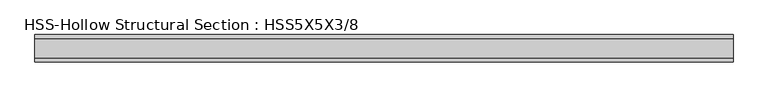
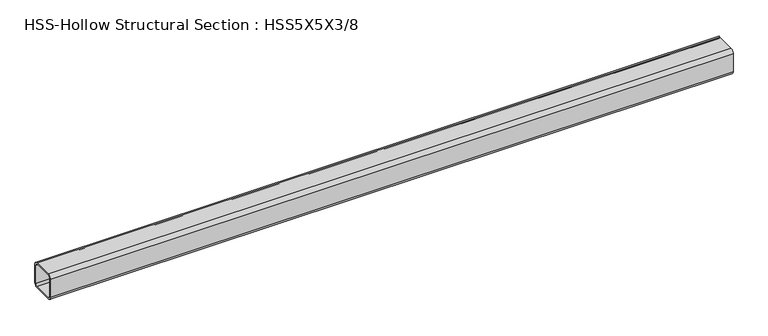
"""IFC4 building model written with IfcOpenShell, lengths in millimetres: member geometry, HSS-Hollow Structural Section : HSS5X5X3/8."""

from ifc_helpers import new_model, si_unit, point, frame, frame_2d, origin, place, context, project, spatial, polyline, circle_curve, trimmed, segment, composite_curve, outline, extrude, source, transform, mapped, element, save


def hss_hollow_structural_section_hss5x5x3_8_3ac4091e(model_context):
    return source(origin(), model_context, "Body", "SweptSolid", [
        extrude(outline(composite_curve([segment(polyline([(63.5, 45.7708), (63.5, -45.7708)]), True, "CONTINUOUS"), segment(trimmed(circle_curve(frame_2d((45.7708, -45.7708)), 17.7292), [point((63.5, -45.7708))], [point((45.7708, -63.5))], False, "CARTESIAN"), True, "CONTINUOUS"), segment(polyline([(45.7708, -63.5), (-45.7708, -63.5)]), True, "CONTINUOUS"), segment(trimmed(circle_curve(frame_2d((-45.7708, -45.7708)), 17.7292), [point((-45.7708, -63.5))], [point((-63.5, -45.7708))], False, "CARTESIAN"), True, "CONTINUOUS"), segment(polyline([(-63.5, -45.7708), (-63.5, 45.7708)]), True, "CONTINUOUS"), segment(trimmed(circle_curve(frame_2d((-45.7708, 45.7708)), 17.7292), [point((-63.5, 45.7708))], [point((-45.7708, 63.5))], False, "CARTESIAN"), True, "CONTINUOUS"), segment(polyline([(-45.7708, 63.5), (45.7708, 63.5)]), True, "CONTINUOUS"), segment(trimmed(circle_curve(frame_2d((45.7708, 45.7708)), 17.7292), [point((45.7708, 63.5))], [point((63.5, 45.7708))], False, "CARTESIAN"), True, "CONTINUOUS")], self_intersect=False), holes=[composite_curve([segment(trimmed(circle_curve(frame_2d((-45.7708, 45.7708)), 8.8646), [point((-45.7708, 54.6354))], [point((-54.6354, 45.7708))], True, "CARTESIAN"), True, "CONTINUOUS"), segment(polyline([(-54.6354, 45.7708), (-54.6354, -45.7708)]), True, "CONTINUOUS"), segment(trimmed(circle_curve(frame_2d((-45.7708, -45.7708)), 8.8646), [point((-54.6354, -45.7708))], [point((-45.7708, -54.6354))], True, "CARTESIAN"), True, "CONTINUOUS"), segment(polyline([(-45.7708, -54.6354), (45.7708, -54.6354)]), True, "CONTINUOUS"), segment(trimmed(circle_curve(frame_2d((45.7708, -45.7708)), 8.8646), [point((45.7708, -54.6354))], [point((54.6354, -45.7708))], True, "CARTESIAN"), True, "CONTINUOUS"), segment(polyline([(54.6354, -45.7708), (54.6354, 45.7708)]), True, "CONTINUOUS"), segment(trimmed(circle_curve(frame_2d((45.7708, 45.7708)), 8.8646), [point((54.6354, 45.7708))], [point((45.7708, 54.6354))], True, "CARTESIAN"), True, "CONTINUOUS"), segment(polyline([(45.7708, 54.6354), (-45.7708, 54.6354)]), True, "CONTINUOUS")], self_intersect=False)]), frame((-1605.4242009, 0.0, 0.0), z_axis=(1.0, 0.0, 0.0), x_axis=(0.0, 1.0, 0.0)), (0.0, 0.0, 1.0), 3260.841735),
    ])


if __name__ == "__main__":
    model = new_model("IFC4")
    model_context = context("Model", 3, world=origin())
    ifc_project = project(units=[si_unit("LENGTHUNIT", "METRE", prefix="MILLI")], contexts=[model_context])
    site = spatial("IfcSite", under=ifc_project)
    building = spatial("IfcBuilding", under=site)
    placement = place(None, origin())
    hss_hollow_structural_section_hss5x5x3_8_shape = hss_hollow_structural_section_hss5x5x3_8_3ac4091e(model_context)
    element("IfcMember", 1, ObjectType="HSS-Hollow Structural Section : HSS5X5X3/8", at=placement, inside=building, context=model_context, shape_type="MappedRepresentation", body=[
        mapped(hss_hollow_structural_section_hss5x5x3_8_shape, transform((0.0, 0.0, 0.0), x_axis=(1.0, 0.0, 0.0), y_axis=(0.0, 1.0, 0.0), z_axis=(0.0, 0.0, 1.0))),
    ])
    save(model, "model.ifc")

# Revit data of these elements
# Type "HSS-Hollow Structural Section : HSS5X5X3/8"
#   Assembly Code = "B10"
#   Shape = "Square"
#   W = 22.3
#   Ht = 0' - 5"
#   Length [instance default] = 5' - 0"
#   b = 0' - 5"
#   kr = 0' - 0.698"
#   t = 0' - 0.349"
#   A = 0.0429167 SF
#   Structural Material [instance default] = Steel ASTM A500, Grade B, Rectangular and Square
# Element 1 (IfcMember, "HSS-Hollow Structural Section : HSS5X5X3/8")
#   Materials on its faces: "Steel ASTM A500, Grade B, Rectangular and Square"
# Materials
#   "Steel ASTM A500, Grade B, Rectangular and Square": class "Metal", colour RGB 199 199 199, transparency 0, Description = "Carbon steel", Cost = 0
